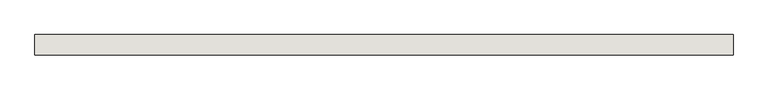
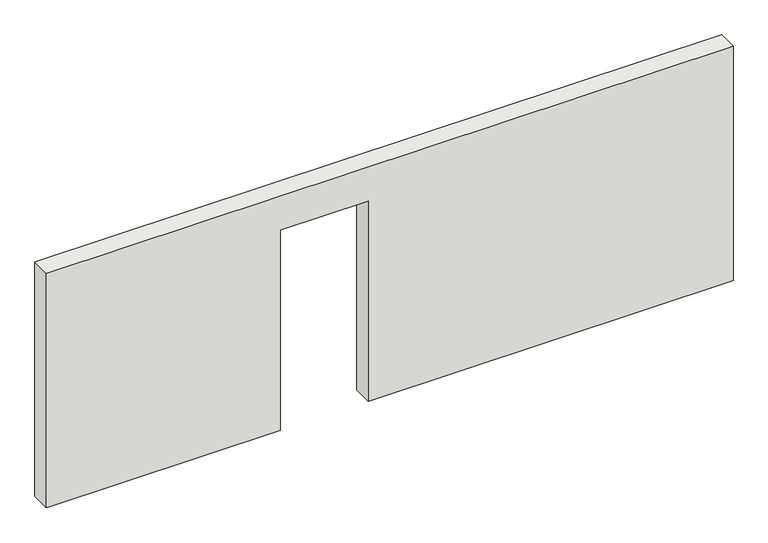
"""IFC4 building model written with IfcOpenShell, lengths in millimetres: wall geometry, Holzwand."""

from ifc_helpers import new_model, si_unit, frame, origin, place, context, project, spatial, polyline, outline, extrude, source, transform, mapped, element, save


def wall_8a9e122a(model_context):
    return source(origin(), model_context, "Body", "SweptSolid", [
        extrude(outline(polyline([(2135.0, 3245.0), (0.0, 3245.0), (0.0, 6925.0), (2500.0, 6925.0), (2500.0, 0.0), (0.0, 0.0), (0.0, 2360.0), (2135.0, 2360.0), (2135.0, 3245.0)])), frame((0.0, 0.0, 0.0), z_axis=(0.0, 1.0, 0.0), x_axis=(0.0, 0.0, 1.0)), (0.0, 0.0, 1.0), 200.0),
    ])


if __name__ == "__main__":
    model = new_model("IFC4")
    model_context = context("Model", 3, world=origin())
    ifc_project = project(units=[si_unit("LENGTHUNIT", "METRE", prefix="MILLI")], contexts=[model_context])
    site = spatial("IfcSite", under=ifc_project)
    building = spatial("IfcBuilding", under=site)
    placement = place(None, origin())
    wall_shape = wall_8a9e122a(model_context)
    element("IfcWall", 1, ObjectType="Holzwand", at=placement, inside=building, context=model_context, shape_type="MappedRepresentation", body=[
        mapped(wall_shape, transform((0.0, 0.0, 0.0), x_axis=(1.0, 0.0, 0.0), y_axis=(0.0, 1.0, 0.0), z_axis=(0.0, 0.0, 1.0))),
    ])
    save(model, "model.ifc")

# Revit data of these elements
# Element 1 (IfcWall, "Holzwand")
#   Materials on its faces: "holzschalung"
# Materials
#   "holzschalung": class "Unassigned", colour RGB 128 128 128, transparency 0
